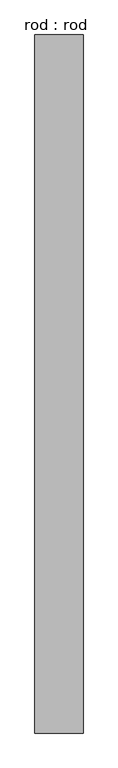
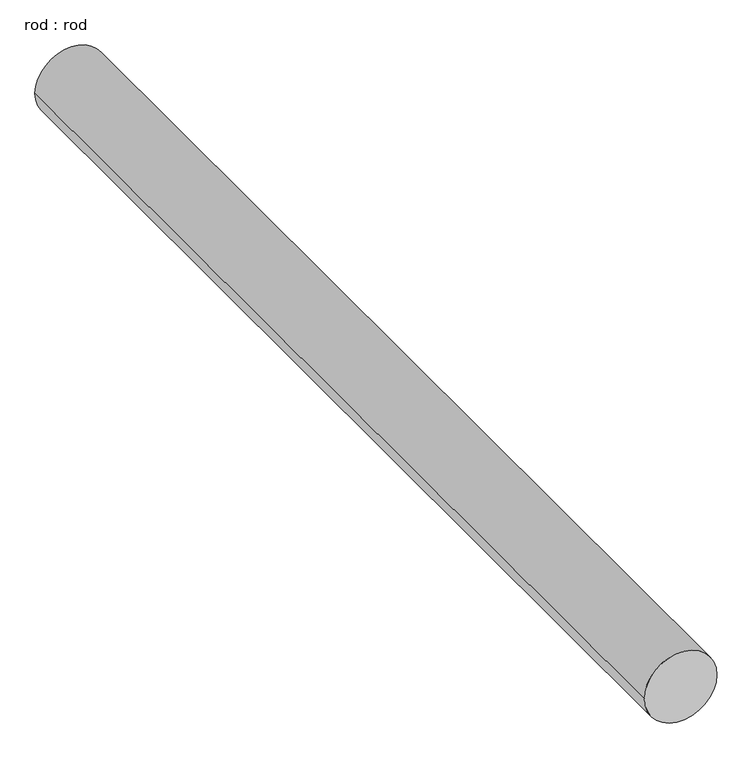
"""IFC4 building model written with IfcOpenShell, lengths in millimetres: proxy geometry, rod : rod."""

from ifc_helpers import new_model, si_unit, point, frame, frame_2d, origin, place, context, project, spatial, circle_curve, trimmed, segment, composite_curve, outline, extrude, source, transform, mapped, element, save


def rod_rod_5aec6dac(model_context):
    return source(origin(), model_context, "Body", "SweptSolid", [
        extrude(outline(composite_curve([segment(trimmed(circle_curve(frame_2d((0.0108462, 0.0)), 200.0), [point((0.0108462, 200.0))], [point((0.0108462, -200.0))], False, "CARTESIAN"), True, "CONTINUOUS"), segment(trimmed(circle_curve(frame_2d((0.0108462, 0.0)), 200.0), [point((0.0108462, -200.0))], [point((0.0108462, 200.0))], False, "CARTESIAN"), True, "CONTINUOUS")], self_intersect=False)), frame((0.0, 1189.1835704, 0.0), z_axis=(0.0, 1.0, 0.0), x_axis=(0.0, 0.0, 1.0)), (0.0, 0.0, 1.0), 5807.0900899),
    ])


if __name__ == "__main__":
    model = new_model("IFC4")
    model_context = context("Model", 3, world=origin())
    ifc_project = project(units=[si_unit("LENGTHUNIT", "METRE", prefix="MILLI")], contexts=[model_context])
    site = spatial("IfcSite", under=ifc_project)
    building = spatial("IfcBuilding", under=site)
    placement = place(None, origin())
    rod_rod_shape = rod_rod_5aec6dac(model_context)
    element("IfcBuildingElementProxy", 1, Name="rod : rod", ObjectType="rod : rod", at=placement, inside=building, context=model_context, shape_type="MappedRepresentation", body=[
        mapped(rod_rod_shape, transform((0.0, 0.0, 0.0), x_axis=(1.0, 0.0, 0.0), y_axis=(0.0, 1.0, 0.0), z_axis=(0.0, 0.0, 1.0))),
    ])
    save(model, "model.ifc")

# Revit data of these elements
# Type "rod : rod"
#   Default Elevation = 0
